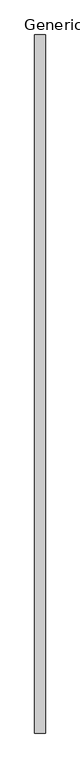
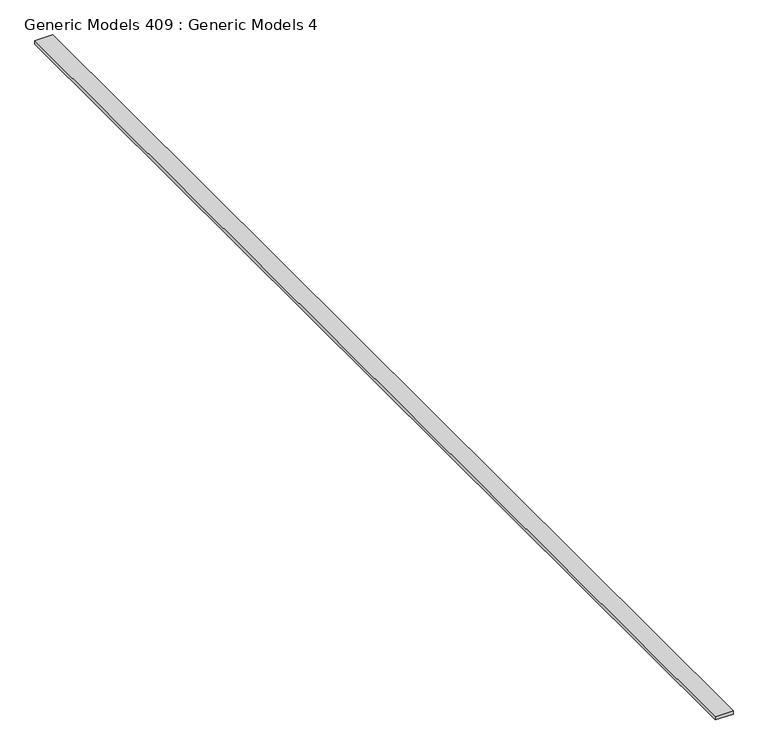
"""IFC4 building model written with IfcOpenShell, lengths in millimetres: proxy geometry, Generic Models 409 : Generic Models 4."""

from ifc_helpers import new_model, si_unit, frame, origin, place, context, project, spatial, polyline, outline, extrude, source, transform, mapped, element, save


def generic_models_409_generic_models_4_f7cc684c(model_context):
    return source(origin(), model_context, "Body", "SweptSolid", [
        extrude(outline(polyline([(-6356.5236296, -6864.9230338), (-6453.8193756, -6864.9230338), (-6453.8193756, -464.1230338), (-6356.5236296, -464.1230338), (-6356.5236296, -6864.9230338)])), frame((0.0, 0.0, 129095.246), z_axis=(0.0, 0.0, 1.0), x_axis=(1.0, 0.0, 0.0)), (0.0, 0.0, 1.0), 18.9872466),
    ])


if __name__ == "__main__":
    model = new_model("IFC4")
    model_context = context("Model", 3, world=origin())
    ifc_project = project(units=[si_unit("LENGTHUNIT", "METRE", prefix="MILLI")], contexts=[model_context])
    site = spatial("IfcSite", under=ifc_project)
    building = spatial("IfcBuilding", under=site)
    placement = place(None, origin())
    generic_models_409_generic_models_4_shape = generic_models_409_generic_models_4_f7cc684c(model_context)
    element("IfcBuildingElementProxy", 1, Name="Generic Models 409 : Generic Models 4", ObjectType="Generic Models 409 : Generic Models 4", at=placement, inside=building, context=model_context, shape_type="MappedRepresentation", body=[
        mapped(generic_models_409_generic_models_4_shape, transform((0.0, 0.0, 0.0), x_axis=(1.0, 0.0, 0.0), y_axis=(0.0, 1.0, 0.0), z_axis=(0.0, 0.0, 1.0))),
    ])
    save(model, "model.ifc")

# Revit data of these elements
# Element 1 (IfcBuildingElementProxy, "Generic Models 409 : Generic Models 4")
#   Materials on its faces: "_HARDWOOD VENEER PLYWOOD (GRADE B, OR BETTER) - MATCH SOLID TRIM SPECIES"
# Materials
#   "_HARDWOOD VENEER PLYWOOD (GRADE B, OR BETTER) - MATCH SOLID TRIM SPECIES": class "Generic", colour RGB 177 130 114, transparency 0, Cost = 0
